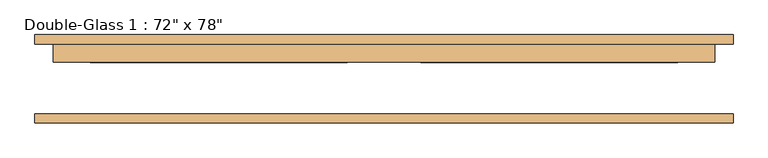
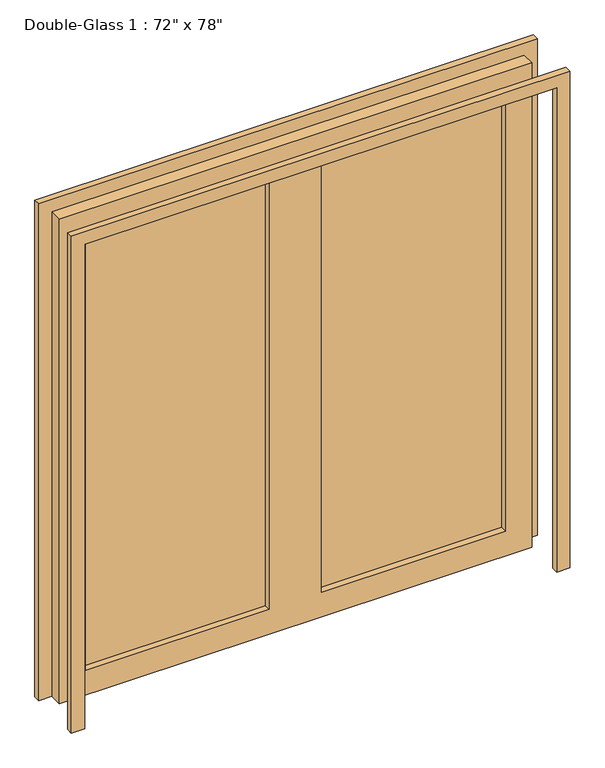
"""IFC4 building model written with IfcOpenShell, lengths in millimetres: door geometry."""

from ifc_helpers import new_model, si_unit, frame, origin, place, context, project, spatial, polyline, outline, extrude, source, transform, mapped, element, save


def door_cbe0d2cf(model_context):
    return source(origin(), model_context, "Body", "SweptSolid", [
        extrude(outline(polyline([(0.0, 965.2), (2032.0, 965.2), (2032.0, -965.2), (0.0, -965.2), (0.0, -914.4), (1981.2, -914.4), (1981.2, 914.4), (0.0, 914.4), (0.0, 965.2)])), frame((0.0, -119.85625, 0.0), z_axis=(0.0, 1.0, 0.0), x_axis=(0.0, 0.0, 1.0)), (0.0, 0.0, 1.0), 25.4),
        extrude(outline(polyline([(1981.2, 914.4), (0.0, 914.4), (0.0, 965.2), (2032.0, 965.2), (2032.0, -965.2), (0.0, -965.2), (0.0, -914.4), (1981.2, -914.4), (1981.2, 914.4)])), frame((0.0, 99.21875, 0.0), z_axis=(0.0, 1.0, 0.0), x_axis=(0.0, 0.0, 1.0)), (0.0, 0.0, 1.0), 25.4),
        extrude(outline(polyline([(812.8, 73.81875), (101.6, 73.81875), (101.6, 80.9625), (812.8, 80.9625), (812.8, 73.81875)])), frame((0.0, 0.0, 101.6), z_axis=(0.0, 0.0, 1.0), x_axis=(1.0, 0.0, 0.0)), (0.0, 0.0, 1.0), 1778.0),
        extrude(outline(polyline([(-101.6, 73.81875), (-812.8, 73.81875), (-812.8, 80.9625), (-101.6, 80.9625), (-101.6, 73.81875)])), frame((0.0, 0.0, 101.6), z_axis=(0.0, 0.0, 1.0), x_axis=(1.0, 0.0, 0.0)), (0.0, 0.0, 1.0), 1778.0),
        extrude(outline(polyline([(1981.2, 914.4), (1981.2, -914.4), (0.0, -914.4), (0.0, 914.4), (1981.2, 914.4)]), holes=[polyline([(1879.6, -101.6), (101.6, -101.6), (101.6, -812.8), (1879.6, -812.8), (1879.6, -101.6)]), polyline([(1879.6, 812.8), (101.6, 812.8), (101.6, 101.6), (1879.6, 101.6), (1879.6, 812.8)])]), frame((0.0, 48.41875, 0.0), z_axis=(0.0, 1.0, 0.0), x_axis=(0.0, 0.0, 1.0)), (0.0, 0.0, 1.0), 50.8),
    ])


if __name__ == "__main__":
    model = new_model("IFC4")
    model_context = context("Model", 3, world=origin())
    ifc_project = project(units=[si_unit("LENGTHUNIT", "METRE", prefix="MILLI")], contexts=[model_context])
    site = spatial("IfcSite", under=ifc_project)
    building = spatial("IfcBuilding", under=site)
    placement = place(None, origin())
    door_shape = door_cbe0d2cf(model_context)
    element("IfcDoor", 1, ObjectType="Double-Glass 1 : 72\" x 78\"", at=placement, inside=building, context=model_context, shape_type="MappedRepresentation", body=[
        mapped(door_shape, transform((0.0, 0.0, 0.0), x_axis=(1.0, 0.0, 0.0), y_axis=(0.0, 1.0, 0.0), z_axis=(0.0, 0.0, 1.0))),
    ])
    save(model, "model.ifc")

# Revit data of these elements
# Type "Double-Glass 1 : 72\" x 78\""
#   Type Mark = "32"
#   Assembly Code = "C1020"
#   Thickness = 0' - 2"
#   Height = 6' - 6"
#   Rail Width - Base = 0' - 4"
#   Rail Width - Top = 0' - 4"
#   Stile Width - Hinge = 0' - 4"
#   Stile Width - Latch = 0' - 4"
#   Trim Projection = 0' - 1"
#   Trim Width = 0' - 2"
#   Width = 6' - 0"
#   Define Thermal Properties by = 0
#   Function = 0
#   Door Material = Door - Panel
#   Frame Material = Door - Frame
#   Wall Closure = (empty or 0)
# Element 1 (IfcDoor, "Double-Glass 1 : 72\" x 78\"")
#   Materials on its faces: "Door - Frame", "Door - Panel", "Glass"
# Materials
#   "Door - Panel": class "Wood", colour RGB 227 170 128, transparency 0, Cost = 0
#   "Door - Frame": class "Miscellaneous", colour RGB 153 76 43, transparency 0, Cost = 0
#   "Glass": class "Glass", colour RGB 236 240 239, transparency 0.5, Description = "Soda Lime Glass", Cost = 0
